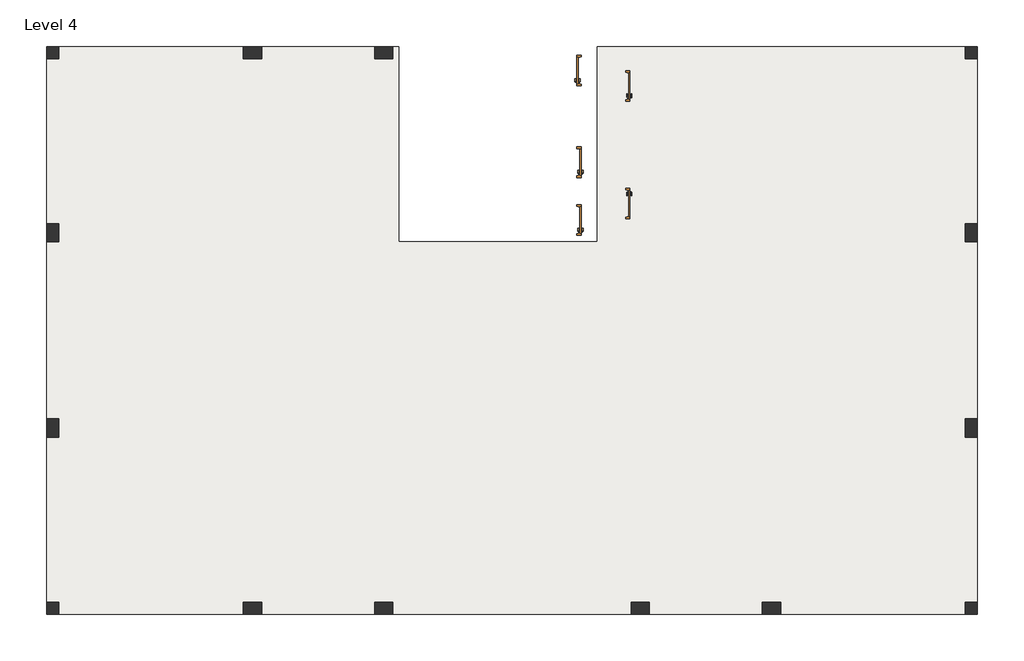
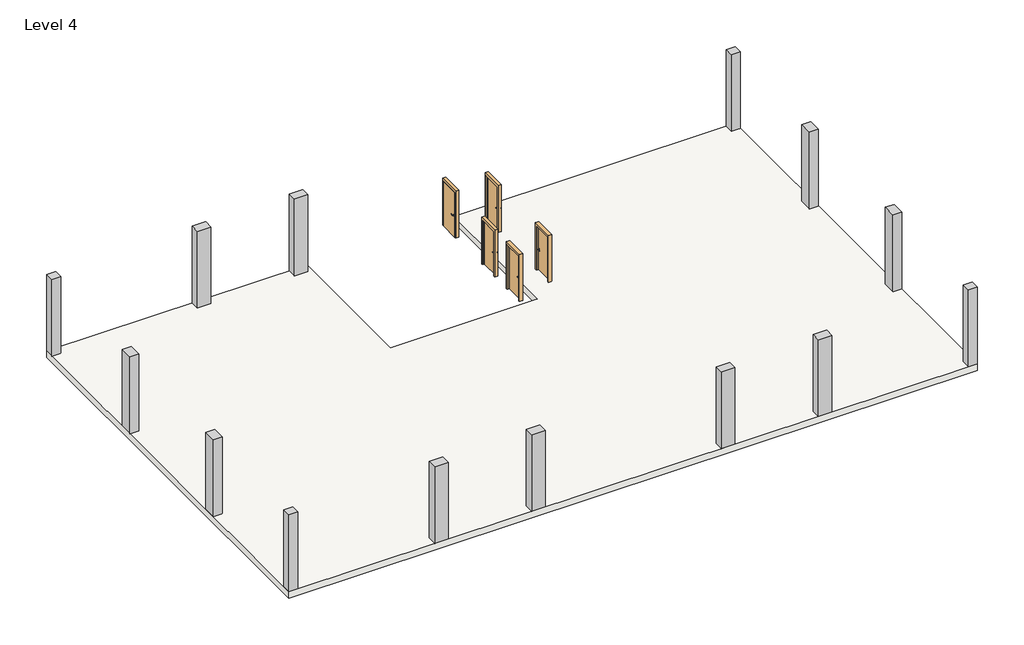
# One storey: 14 columns, 5 doors, 1 slab.
"""IFC4 building model written with IfcOpenShell, lengths in millimetres."""

import ifcopenshell
import ifcopenshell.guid

model = None  # the IFC model being written
_history = None  # IfcOwnerHistory: only IFC2X3 demands one
_inside = {}  # id of a spatial element -> (the spatial element, [elements in it])
_under = {}  # id of a project, library or spatial element -> (it, [spatial elements below it])
_declared = {}  # id of a project -> (the project, [libraries it declares])
_typed = {}  # id of a type object -> (the type object, [elements of that type])
_made_of = {}  # id of a material, layer set ... -> (it, [elements and type objects made of it])


def new_model(schema):
    """Start an empty IFC model of exactly this schema.

    Asked for "IFC4X3", IfcOpenShell would pick the latest addendum, in which some entities
    have other attributes; the version numbers below select the first issue.
    IFC2X3 requires an IfcOwnerHistory on every rooted entity: one is made here for all.
    """
    global model, _history
    if schema == "IFC4X3":
        model = ifcopenshell.file(schema_version=(4, 3, 0, 0))
    else:
        model = ifcopenshell.file(schema=schema)
    _inside.clear()
    _under.clear()
    _declared.clear()
    _typed.clear()
    _made_of.clear()
    _history = None
    if model.schema == "IFC2X3":
        org = make("IfcOrganization", Name="unknown")
        user = make(
            "IfcPersonAndOrganization",
            ThePerson=make("IfcPerson", FamilyName="unknown"),
            TheOrganization=org,
        )
        app = make(
            "IfcApplication",
            ApplicationDeveloper=org,
            Version="unknown",
            ApplicationFullName="unknown",
            ApplicationIdentifier="unknown",
        )
        _history = make(
            "IfcOwnerHistory",
            OwningUser=user,
            OwningApplication=app,
            ChangeAction="ADDED",
            CreationDate=0,
        )
    return model


def make(cls, **values):
    """One entity of the class cls with the attributes given. An attribute that is None is left unset."""
    return model.create_entity(
        cls, **{name: value for name, value in values.items() if value is not None}
    )


def rooted(cls, **values):
    """An entity with a GlobalId (a new one), such as an element, a storey or a relation."""
    return make(cls, GlobalId=ifcopenshell.guid.new(), OwnerHistory=_history, **values)


def si_unit(unit_type, name, prefix=None):
    """IfcSIUnit, for example si_unit("LENGTHUNIT", "METRE", prefix="MILLI")."""
    return make("IfcSIUnit", UnitType=unit_type, Prefix=prefix, Name=name)


def assignment(units):
    """IfcUnitAssignment: the units of a project."""
    return None if units is None else make("IfcUnitAssignment", Units=units)


def point(xyz):
    """IfcCartesianPoint."""
    return None if xyz is None else make("IfcCartesianPoint", Coordinates=xyz)


def direction(xyz):
    """IfcDirection."""
    return None if xyz is None else make("IfcDirection", DirectionRatios=xyz)


def frame(location, z_axis=None, x_axis=None):
    """IfcAxis2Placement3D, a coordinate frame: its origin and axes. An axis left out is left unset."""
    return make(
        "IfcAxis2Placement3D",
        Location=point(location),
        Axis=direction(z_axis),
        RefDirection=direction(x_axis),
    )


def frame_2d(location, x_axis=None):
    """IfcAxis2Placement2D, a coordinate frame in the plane: its origin and x axis."""
    return make(
        "IfcAxis2Placement2D", Location=point(location), RefDirection=direction(x_axis)
    )


def origin():
    """The frame at (0, 0, 0) with its axes left unset."""
    return frame((0.0, 0.0, 0.0))


def origin_with_axes():
    """The frame at (0, 0, 0) with the z axis (0, 0, 1) and the x axis (1, 0, 0) written out."""
    return frame((0.0, 0.0, 0.0), z_axis=(0.0, 0.0, 1.0), x_axis=(1.0, 0.0, 0.0))


def place(relative_to, where):
    """IfcLocalPlacement: puts the frame where relative to a parent placement (None: the world)."""
    return make(
        "IfcLocalPlacement", PlacementRelTo=relative_to, RelativePlacement=where
    )


def context(
    kind, dimensions, precision=None, world=None, true_north=None, identifier=None
):
    """IfcGeometricRepresentationContext, for example the 3D "Model" context."""
    return make(
        "IfcGeometricRepresentationContext",
        ContextIdentifier=identifier,
        ContextType=kind,
        CoordinateSpaceDimension=dimensions,
        Precision=precision,
        WorldCoordinateSystem=world,
        TrueNorth=true_north,
    )


def project(units=None, contexts=None):
    """IfcProject with its units and contexts."""
    return rooted(
        "IfcProject",
        Name="project",
        RepresentationContexts=contexts,
        UnitsInContext=assignment(units),
    )


def spatial(cls, under=None, at=None, **own):
    """A site, building, storey or space (cls), placed at a placement, below another one or the project."""
    s = rooted(cls, ObjectPlacement=at, **own)
    if under is not None:
        _under.setdefault(under.id(), (under, []))[1].append(s)
    return s


def polyline(points):
    """IfcPolyline through the points."""
    return make("IfcPolyline", Points=[point(p) for p in points])


def circle_curve(where, radius):
    """IfcCircle in the frame where."""
    return make("IfcCircle", Position=where, Radius=radius)


def ellipse_curve(where, semi_axis1, semi_axis2):
    """IfcEllipse in the frame where."""
    return make(
        "IfcEllipse", Position=where, SemiAxis1=semi_axis1, SemiAxis2=semi_axis2
    )


def trimmed(basis, trim1, trim2, sense, master):
    """IfcTrimmedCurve: the piece of a basis curve between two trims."""
    return make(
        "IfcTrimmedCurve",
        BasisCurve=basis,
        Trim1=trim1,
        Trim2=trim2,
        SenseAgreement=sense,
        MasterRepresentation=master,
    )


def segment(curve, same_sense, transition):
    """IfcCompositeCurveSegment."""
    return make(
        "IfcCompositeCurveSegment",
        Transition=transition,
        SameSense=same_sense,
        ParentCurve=curve,
    )


def composite_curve(segments, self_intersect=None):
    """IfcCompositeCurve: segments joined end to end."""
    return make("IfcCompositeCurve", Segments=segments, SelfIntersect=self_intersect)


def outline(outer, holes=None, kind="AREA"):
    """IfcArbitraryClosedProfileDef: a profile drawn as a closed curve; with holes, ...WithVoids."""
    if holes is None:
        return make("IfcArbitraryClosedProfileDef", ProfileType=kind, OuterCurve=outer)
    return make(
        "IfcArbitraryProfileDefWithVoids",
        ProfileType=kind,
        OuterCurve=outer,
        InnerCurves=holes,
    )


def extrude(swept, where, along, depth):
    """IfcExtrudedAreaSolid: the profile swept, set in the frame where, extruded along a direction by depth."""
    return make(
        "IfcExtrudedAreaSolid",
        SweptArea=swept,
        Position=where,
        ExtrudedDirection=direction(along),
        Depth=depth,
    )


def faces_of(points, faces, orient=None, outer=None):
    """IfcFace entities. A face is a list of loops; a loop is a list of indices into points, from 0.

    orient and outer hold one flag for each loop. By default every Orientation is true, the
    first loop of a face is its IfcFaceOuterBound and the others are IfcFaceBound.
    """
    made = []
    for i, loops in enumerate(faces):
        bounds = []
        for j, loop in enumerate(loops):
            is_outer = j == 0 if outer is None else outer[i][j]
            bounds.append(
                make(
                    "IfcFaceOuterBound" if is_outer else "IfcFaceBound",
                    Bound=make("IfcPolyLoop", Polygon=[points[k] for k in loop]),
                    Orientation=True if orient is None else orient[i][j],
                )
            )
        made.append(make("IfcFace", Bounds=bounds))
    return made


def faceted_brep(points, faces, orient=None, outer=None, voids=None):
    """IfcFacetedBrep: a solid bounded by flat faces; with voids (closed shells), ...WithVoids."""
    shared = [point(p) for p in points]
    hull = make("IfcClosedShell", CfsFaces=faces_of(shared, faces, orient, outer))
    if voids is None:
        return make("IfcFacetedBrep", Outer=hull)
    return make(
        "IfcFacetedBrepWithVoids",
        Outer=hull,
        Voids=[
            make(cls, CfsFaces=faces_of(shared, fs, o, b)) for cls, fs, o, b in voids
        ],
    )


def shape(context_of_items, identifier, shape_type, items):
    """IfcShapeRepresentation: the items that make up one representation, for example the "Body"."""
    return make(
        "IfcShapeRepresentation",
        ContextOfItems=context_of_items,
        RepresentationIdentifier=identifier,
        RepresentationType=shape_type,
        Items=items,
    )


def source(mapping_origin, context_of_items, identifier, shape_type, items):
    """IfcRepresentationMap: a shape defined once, which mapped items show again and again."""
    return make(
        "IfcRepresentationMap",
        MappingOrigin=mapping_origin,
        MappedRepresentation=shape(context_of_items, identifier, shape_type, items),
    )


def transform(
    local_origin,
    x_axis=None,
    y_axis=None,
    z_axis=None,
    scale=None,
    scale2=None,
    scale3=None,
    uniform=True,
):
    """IfcCartesianTransformationOperator3D, or its non-uniform kind. x_axis, y_axis, z_axis: its Axis1, 2, 3."""
    if uniform:
        return make(
            "IfcCartesianTransformationOperator3D",
            Axis1=direction(x_axis),
            Axis2=direction(y_axis),
            LocalOrigin=point(local_origin),
            Scale=scale,
            Axis3=direction(z_axis),
        )
    return make(
        "IfcCartesianTransformationOperator3DnonUniform",
        Axis1=direction(x_axis),
        Axis2=direction(y_axis),
        LocalOrigin=point(local_origin),
        Scale=scale,
        Axis3=direction(z_axis),
        Scale2=scale2,
        Scale3=scale3,
    )


def mapped(mapping_source, mapping_target):
    """IfcMappedItem: shows the shape of a source again, moved by a transform."""
    return make(
        "IfcMappedItem", MappingSource=mapping_source, MappingTarget=mapping_target
    )


def made_of(thing, what):
    """Note that an element or type object is made of a material, layer set ...; save() writes the relation."""
    if what is not None:
        _made_of.setdefault(what.id(), (what, []))[1].append(thing)
    return thing


def element(
    cls,
    number,
    at=None,
    inside=None,
    cuts=None,
    type_object=None,
    material=None,
    context=None,
    identifier="Body",
    shape_type=None,
    held_by="IfcProductDefinitionShape",
    body=None,
    shapes=None,
    **own,
):
    """One element of the class cls, such as IfcWall. Its Tag is "e" and its number.

    at: its placement. inside: the storey or other place that contains it. cuts: it is an
    opening in that element (IfcRelVoidsElement). A single representation is given by context,
    identifier, shape_type and body (its items); several are given by shapes. held_by: the class
    of the entity that holds the representations. save() writes the other relations.
    """
    e = rooted(cls, Tag="e%d" % number, ObjectPlacement=at, **own)
    if body is not None:
        shapes = [shape(context, identifier, shape_type, body)]
    if shapes is not None:
        e.Representation = make(held_by, Representations=shapes)
    if inside is not None:
        _inside.setdefault(inside.id(), (inside, []))[1].append(e)
    if cuts is not None:
        rooted(
            "IfcRelVoidsElement", RelatingBuildingElement=cuts, RelatedOpeningElement=e
        )
    if type_object is not None:
        _typed.setdefault(type_object.id(), (type_object, []))[1].append(e)
    return made_of(e, material)


def aggregate(whole, parts):
    """IfcRelAggregates: a whole, such as a stair, and the parts it consists of."""
    return rooted("IfcRelAggregates", RelatingObject=whole, RelatedObjects=parts)


def save(model, path):
    """Write the relations noted so far, then the file.

    IfcRelAggregates (storeys below a building ...), IfcRelContainedInSpatialStructure (elements
    in a storey), IfcRelDefinesByType, IfcRelAssociatesMaterial and IfcRelDeclares: one each for
    every whole, place, type object, material and project.
    """
    for whole, parts in _under.values():
        aggregate(whole, parts)
    for where, things in _inside.values():
        rooted(
            "IfcRelContainedInSpatialStructure",
            RelatedElements=things,
            RelatingStructure=where,
        )
    for kind, things in _typed.values():
        rooted("IfcRelDefinesByType", RelatedObjects=things, RelatingType=kind)
    for what, things in _made_of.values():
        rooted("IfcRelAssociatesMaterial", RelatedObjects=things, RelatingMaterial=what)
    for by, libraries in _declared.values():
        rooted("IfcRelDeclares", RelatingContext=by, RelatedDefinitions=libraries)
    model.write(path)


def plane_surface(at):
    """IfcPlane: the flat surface through the origin of the frame at, square to its z axis."""
    return make("IfcPlane", Position=at)


def cylinder_surface(at, radius):
    """IfcCylindricalSurface: all points at the distance radius from the z axis of the frame at."""
    return make("IfcCylindricalSurface", Position=at, Radius=radius)


def revolved_surface(curve, axis_point, axis_direction):
    """IfcSurfaceOfRevolution: the curve turned about the line through axis_point along axis_direction."""
    return make(
        "IfcSurfaceOfRevolution",
        SweptCurve=make("IfcArbitraryOpenProfileDef", ProfileType="CURVE", Curve=curve),
        AxisPosition=make("IfcAxis1Placement", Location=point(axis_point), Axis=direction(axis_direction)),
    )


def advanced_brep(points, edges, surfaces, faces):
    """IfcAdvancedBrep: a solid bounded by faces that lie on surfaces and meet in shared edges.

    An edge is (start, end): straight between two places in points (the first is 0);
    or (start, end, curve); or (start, end, curve, False) where it runs against its curve.
    A face is (place in surfaces, loops), or (place, loops, False) where it looks against
    its surface's normal. A loop lists edges by number (the first is 1), with a minus sign
    where the edge is run from its end to its start. The first loop is the outer one.
    """
    corners = [point(p) for p in points]
    vertices = [make("IfcVertexPoint", VertexGeometry=c) for c in corners]
    made = []
    for start, end, *more in edges:
        made.append(
            make(
                "IfcEdgeCurve",
                EdgeStart=vertices[start],
                EdgeEnd=vertices[end],
                EdgeGeometry=more[0] if more else make("IfcPolyline", Points=[corners[start], corners[end]]),
                SameSense=more[1] if len(more) > 1 else True,
            )
        )
    hull = []
    for where, loops, *sense in faces:
        bounds = []
        for j, loop in enumerate(loops):
            ring = [make("IfcOrientedEdge", EdgeElement=made[abs(k) - 1], Orientation=k > 0) for k in loop]
            bounds.append(
                make(
                    "IfcFaceOuterBound" if j == 0 else "IfcFaceBound",
                    Bound=make("IfcEdgeLoop", EdgeList=ring),
                    Orientation=True,
                )
            )
        hull.append(make("IfcAdvancedFace", Bounds=bounds, FaceSurface=surfaces[where], SameSense=sense[0] if sense else True))
    return make("IfcAdvancedBrep", Outer=make("IfcClosedShell", CfsFaces=hull))


def door_9f6fe377(model_context):
    return source(origin(), model_context, "Body", "SolidModel", [
        advanced_brep(
        [(-392.190625, -25.3375, 1016.0), (-372.190625, -25.3375, 1016.0), (-392.190625, 4.6625, 1016.0), (-372.190625, 4.6625, 1016.0), (-367.190625, 9.6625, 1016.0), (-367.190625, 29.6625, 1016.0), (-262.190625, 29.6625, 1016.0), (-262.190625, 9.6625, 1016.0)],
        [
            (0, 1, circle_curve(frame((-382.190625, -25.3375, 1016.0), z_axis=(0.0, -1.0, 0.0), x_axis=(1.0, 0.0, 0.0)), 10.0)),
            (1, 0, circle_curve(frame((-382.190625, -25.3375, 1016.0), z_axis=(0.0, -1.0, 0.0), x_axis=(1.0, 0.0, 0.0)), 10.0)),
            (0, 2),
            (2, 3, circle_curve(frame((-382.190625, 4.6625, 1016.0), z_axis=(0.0, -1.0, 0.0), x_axis=(1.0, 0.0, 0.0)), 10.0)),
            (3, 1),
            (3, 2, circle_curve(frame((-382.190625, 4.6625, 1016.0), z_axis=(0.0, -1.0, 0.0), x_axis=(1.0, 0.0, 0.0)), 10.0)),
            (4, 3, circle_curve(frame((-367.190625, 4.6625, 1016.0), z_axis=(0.0, 0.0, 1.0), x_axis=(-1.0, 0.0, 0.0)), 5.0)),
            (2, 5, circle_curve(frame((-367.190625, 4.6625, 1016.0), z_axis=(0.0, 0.0, -1.0), x_axis=(-1.0, 0.0, 0.0)), 25.0)),
            (5, 4, circle_curve(frame((-367.190625, 19.6625, 1016.0), z_axis=(-1.0, 0.0, 0.0), x_axis=(0.0, -1.0, 0.0)), 10.0)),
            (4, 5, circle_curve(frame((-367.190625, 19.6625, 1016.0), z_axis=(-1.0, 0.0, 0.0), x_axis=(0.0, -1.0, 0.0)), 10.0)),
            (6, 7, circle_curve(frame((-262.190625, 19.6625, 1016.0), z_axis=(1.0, 0.0, 0.0), x_axis=(0.0, -1.0, 0.0)), 10.0)),
            (7, 6, circle_curve(frame((-262.190625, 19.6625, 1016.0), z_axis=(1.0, 0.0, 0.0), x_axis=(0.0, -1.0, 0.0)), 10.0)),
            (5, 6),
            (7, 4),
        ],
        [
            plane_surface(frame((-382.190625, -25.3375, 1016.0), z_axis=(0.0, -1.0, 0.0), x_axis=(0.0, 0.0, 1.0))),
            cylinder_surface(frame((-382.190625, -25.3375, 1016.0), z_axis=(0.0, -1.0, 0.0), x_axis=(1.0, 0.0, 0.0)), 10.0),
            revolved_surface(trimmed(ellipse_curve(frame((-382.190625, 4.6625, 1016.0), z_axis=(0.0, -1.0, 0.0), x_axis=(1.0, 0.0, 0.0)), 10.0, 10.0), [point((-392.190625, 4.6625, 1016.0))], [point((-372.190625, 4.6625, 1016.0))], True, "CARTESIAN"), (-367.190625, 4.6625, 1016.0), (0.0, 0.0, -1.0)),
            revolved_surface(trimmed(ellipse_curve(frame((-382.190625, 4.6625, 1016.0), z_axis=(0.0, -1.0, 0.0), x_axis=(1.0, 0.0, 0.0)), 10.0, 10.0), [point((-372.190625, 4.6625, 1016.0))], [point((-392.190625, 4.6625, 1016.0))], True, "CARTESIAN"), (-367.190625, 4.6625, 1016.0), (0.0, 0.0, -1.0)),
            plane_surface(frame((-262.190625, 19.6625, 1016.0), z_axis=(1.0, 0.0, 0.0), x_axis=(0.0, 0.0, 1.0))),
            cylinder_surface(frame((-367.190625, 19.6625, 1016.0), z_axis=(-1.0, 0.0, 0.0), x_axis=(0.0, -1.0, 0.0)), 10.0),
        ],
        [
            (0, [[1, 2]]),
            (1, [[-1, 3, 4, 5]]),
            (1, [[-2, -5, 6, -3]]),
            (2, [[7, -4, 8, 9]]),
            (3, [[-8, -6, -7, 10]]),
            (4, [[11, 12]]),
            (5, [[-9, 13, -12, 14]]),
            (5, [[-10, -14, -11, -13]]),
        ],
    ),
        extrude(outline(composite_curve([segment(trimmed(circle_curve(frame_2d((1016.0, -384.690625)), 30.0), [point((1016.0, -414.690625))], [point((1016.0, -354.690625))], False, "CARTESIAN"), True, "CONTINUOUS"), segment(trimmed(circle_curve(frame_2d((1016.0, -384.690625)), 30.0), [point((1016.0, -354.690625))], [point((1016.0, -414.690625))], False, "CARTESIAN"), True, "CONTINUOUS")], self_intersect=False)), frame((0.0, -33.3375, 0.0), z_axis=(0.0, 1.0, 0.0), x_axis=(0.0, 0.0, 1.0)), (0.0, 0.0, 1.0), 8.0),
        advanced_brep(
        [(-392.190625, -85.7875, 1016.0), (-372.190625, -85.7875, 1016.0), (-372.190625, -115.7875, 1016.0), (-392.190625, -115.7875, 1016.0), (-367.190625, -120.7875, 1016.0), (-367.190625, -140.7875, 1016.0), (-262.190625, -140.7875, 1016.0), (-262.190625, -120.7875, 1016.0)],
        [
            (0, 1, circle_curve(frame((-382.190625, -85.7875, 1016.0), z_axis=(0.0, 1.0, 0.0), x_axis=(1.0, 0.0, 0.0)), 10.0)),
            (1, 0, circle_curve(frame((-382.190625, -85.7875, 1016.0), z_axis=(0.0, 1.0, 0.0), x_axis=(1.0, 0.0, 0.0)), 10.0)),
            (1, 2),
            (2, 3, circle_curve(frame((-382.190625, -115.7875, 1016.0), z_axis=(0.0, 1.0, 0.0), x_axis=(1.0, 0.0, 0.0)), 10.0)),
            (3, 0),
            (3, 2, circle_curve(frame((-382.190625, -115.7875, 1016.0), z_axis=(0.0, 1.0, 0.0), x_axis=(1.0, 0.0, 0.0)), 10.0)),
            (4, 5, circle_curve(frame((-367.190625, -130.7875, 1016.0), z_axis=(-1.0, 0.0, 0.0), x_axis=(0.0, 1.0, 0.0)), 10.0)),
            (5, 3, circle_curve(frame((-367.190625, -115.7875, 1016.0), z_axis=(0.0, 0.0, -1.0), x_axis=(-1.0, 0.0, 0.0)), 25.0)),
            (2, 4, circle_curve(frame((-367.190625, -115.7875, 1016.0), z_axis=(0.0, 0.0, 1.0), x_axis=(-1.0, 0.0, 0.0)), 5.0)),
            (5, 4, circle_curve(frame((-367.190625, -130.7875, 1016.0), z_axis=(-1.0, 0.0, 0.0), x_axis=(0.0, 1.0, 0.0)), 10.0)),
            (6, 7, circle_curve(frame((-262.190625, -130.7875, 1016.0), z_axis=(1.0, 0.0, 0.0), x_axis=(0.0, 1.0, 0.0)), 10.0)),
            (7, 6, circle_curve(frame((-262.190625, -130.7875, 1016.0), z_axis=(1.0, 0.0, 0.0), x_axis=(0.0, 1.0, 0.0)), 10.0)),
            (4, 7),
            (6, 5),
        ],
        [
            plane_surface(frame((-382.190625, -85.7875, 1016.0), z_axis=(0.0, 1.0, 0.0), x_axis=(0.0, 0.0, 1.0))),
            cylinder_surface(frame((-382.190625, -85.7875, 1016.0), z_axis=(0.0, 1.0, 0.0), x_axis=(1.0, 0.0, 0.0)), 10.0),
            revolved_surface(trimmed(ellipse_curve(frame((-382.190625, -115.7875, 1016.0), z_axis=(0.0, -1.0, 0.0), x_axis=(1.0, 0.0, 0.0)), 10.0, 10.0), [point((-392.190625, -115.7875, 1016.0))], [point((-372.190625, -115.7875, 1016.0))], True, "CARTESIAN"), (-367.190625, -115.7875, 1016.0), (0.0, 0.0, -1.0)),
            revolved_surface(trimmed(ellipse_curve(frame((-382.190625, -115.7875, 1016.0), z_axis=(0.0, -1.0, 0.0), x_axis=(1.0, 0.0, 0.0)), 10.0, 10.0), [point((-372.190625, -115.7875, 1016.0))], [point((-392.190625, -115.7875, 1016.0))], True, "CARTESIAN"), (-367.190625, -115.7875, 1016.0), (0.0, 0.0, -1.0)),
            plane_surface(frame((-262.190625, -130.7875, 1016.0), z_axis=(1.0, 0.0, 0.0), x_axis=(0.0, 0.0, 1.0))),
            cylinder_surface(frame((-367.190625, -130.7875, 1016.0), z_axis=(-1.0, 0.0, 0.0), x_axis=(0.0, 1.0, 0.0)), 10.0),
        ],
        [
            (0, [[1, 2]]),
            (1, [[3, 4, 5, -2]]),
            (1, [[-5, 6, -3, -1]]),
            (2, [[7, 8, -4, 9]]),
            (3, [[10, -9, -6, -8]]),
            (4, [[11, 12]]),
            (5, [[13, -11, 14, -7]]),
            (5, [[-14, -12, -13, -10]]),
        ],
    ),
        extrude(outline(composite_curve([segment(trimmed(circle_curve(frame_2d((1016.0, -384.690625)), 30.0), [point((1016.0, -414.690625))], [point((1016.0, -354.690625))], False, "CARTESIAN"), True, "CONTINUOUS"), segment(trimmed(circle_curve(frame_2d((1016.0, -384.690625)), 30.0), [point((1016.0, -354.690625))], [point((1016.0, -414.690625))], False, "CARTESIAN"), True, "CONTINUOUS")], self_intersect=False)), frame((0.0, -85.7875, 0.0), z_axis=(0.0, 1.0, 0.0), x_axis=(0.0, 0.0, 1.0)), (0.0, 0.0, 1.0), 8.0),
        faceted_brep([(457.2, -28.575, 0.0), (441.325, -28.575, 0.0), (441.325, 19.05, 0.0), (457.2, 19.05, 0.0), (457.2, 68.2625, 0.0), (508.0, 68.2625, 0.0), (508.0, -77.7875, 0.0), (457.2, -77.7875, 0.0), (457.2, -77.7875, 2133.6), (457.2, -28.575, 2133.6), (508.0, -77.7875, 2235.2), (-508.0, -77.7875, 2235.2), (-508.0, -77.7875, 0.0), (-457.2, -77.7875, 0.0), (-457.2, -77.7875, 2133.6), (508.0, 68.2625, 2235.2), (457.2, 68.2625, 2133.6), (-457.2, 68.2625, 2133.6), (-457.2, 68.2625, 0.0), (-508.0, 68.2625, 0.0), (-508.0, 68.2625, 2235.2), (457.2, 19.05, 2133.6), (441.325, 19.05, 2117.725), (-441.325, 19.05, 2117.725), (-441.325, 19.05, 0.0), (-457.2, 19.05, 0.0), (-457.2, 19.05, 2133.6), (441.325, -28.575, 2117.725), (-457.2, -28.575, 2133.6), (-457.2, -28.575, 0.0), (-441.325, -28.575, 0.0), (-441.325, -28.575, 2117.725)], [[[0, 1, 2, 3, 4, 5, 6, 7]], [[7, 8, 9, 0]], [[6, 10, 11, 12, 13, 14, 8, 7]], [[5, 15, 10, 6]], [[4, 16, 17, 18, 19, 20, 15, 5]], [[3, 21, 16, 4]], [[2, 22, 23, 24, 25, 26, 21, 3]], [[1, 27, 22, 2]], [[0, 9, 28, 29, 30, 31, 27, 1]], [[8, 14, 28, 9]], [[16, 21, 26, 17]], [[22, 27, 31, 23]], [[12, 19, 18, 25, 24, 30, 29, 13]], [[13, 29, 28, 14]], [[11, 20, 19, 12]], [[17, 26, 25, 18]], [[23, 31, 30, 24]], [[15, 20, 11, 10]]]),
        extrude(outline(polyline([(457.2, -33.3375), (457.2, -77.7875), (-457.2, -77.7875), (-457.2, -33.3375), (457.2, -33.3375)])), origin_with_axes(), (0.0, 0.0, 1.0), 2133.6),
    ])


def door_87fe937e(model_context):
    return source(origin(), model_context, "Body", "SolidModel", [
        advanced_brep(
        [(-392.190625, 25.3375, 1016.0), (-372.190625, 25.3375, 1016.0), (-372.190625, -4.6625, 1016.0), (-392.190625, -4.6625, 1016.0), (-367.190625, -9.6625, 1016.0), (-367.190625, -29.6625, 1016.0), (-262.190625, -29.6625, 1016.0), (-262.190625, -9.6625, 1016.0)],
        [
            (0, 1, circle_curve(frame((-382.190625, 25.3375, 1016.0), z_axis=(0.0, 1.0, 0.0), x_axis=(1.0, 0.0, 0.0)), 10.0)),
            (1, 0, circle_curve(frame((-382.190625, 25.3375, 1016.0), z_axis=(0.0, 1.0, 0.0), x_axis=(1.0, 0.0, 0.0)), 10.0)),
            (1, 2),
            (2, 3, circle_curve(frame((-382.190625, -4.6625, 1016.0), z_axis=(0.0, 1.0, 0.0), x_axis=(1.0, 0.0, 0.0)), 10.0)),
            (3, 0),
            (3, 2, circle_curve(frame((-382.190625, -4.6625, 1016.0), z_axis=(0.0, 1.0, 0.0), x_axis=(1.0, 0.0, 0.0)), 10.0)),
            (4, 5, circle_curve(frame((-367.190625, -19.6625, 1016.0), z_axis=(-1.0, 0.0, 0.0), x_axis=(0.0, 1.0, 0.0)), 10.0)),
            (5, 3, circle_curve(frame((-367.190625, -4.6625, 1016.0), z_axis=(0.0, 0.0, -1.0), x_axis=(-1.0, 0.0, 0.0)), 25.0)),
            (2, 4, circle_curve(frame((-367.190625, -4.6625, 1016.0), z_axis=(0.0, 0.0, 1.0), x_axis=(-1.0, 0.0, 0.0)), 5.0)),
            (5, 4, circle_curve(frame((-367.190625, -19.6625, 1016.0), z_axis=(-1.0, 0.0, 0.0), x_axis=(0.0, 1.0, 0.0)), 10.0)),
            (6, 7, circle_curve(frame((-262.190625, -19.6625, 1016.0), z_axis=(1.0, 0.0, 0.0), x_axis=(0.0, 1.0, 0.0)), 10.0)),
            (7, 6, circle_curve(frame((-262.190625, -19.6625, 1016.0), z_axis=(1.0, 0.0, 0.0), x_axis=(0.0, 1.0, 0.0)), 10.0)),
            (4, 7),
            (6, 5),
        ],
        [
            plane_surface(frame((-382.190625, 25.3375, 1016.0), z_axis=(0.0, 1.0, 0.0), x_axis=(0.0, 0.0, 1.0))),
            cylinder_surface(frame((-382.190625, 25.3375, 1016.0), z_axis=(0.0, 1.0, 0.0), x_axis=(1.0, 0.0, 0.0)), 10.0),
            revolved_surface(trimmed(ellipse_curve(frame((-382.190625, -4.6625, 1016.0), z_axis=(0.0, -1.0, 0.0), x_axis=(1.0, 0.0, 0.0)), 10.0, 10.0), [point((-392.190625, -4.6625, 1016.0))], [point((-372.190625, -4.6625, 1016.0))], True, "CARTESIAN"), (-367.190625, -4.6625, 1016.0), (0.0, 0.0, -1.0)),
            revolved_surface(trimmed(ellipse_curve(frame((-382.190625, -4.6625, 1016.0), z_axis=(0.0, -1.0, 0.0), x_axis=(1.0, 0.0, 0.0)), 10.0, 10.0), [point((-372.190625, -4.6625, 1016.0))], [point((-392.190625, -4.6625, 1016.0))], True, "CARTESIAN"), (-367.190625, -4.6625, 1016.0), (0.0, 0.0, -1.0)),
            plane_surface(frame((-262.190625, -19.6625, 1016.0), z_axis=(1.0, 0.0, 0.0), x_axis=(0.0, 0.0, 1.0))),
            cylinder_surface(frame((-367.190625, -19.6625, 1016.0), z_axis=(-1.0, 0.0, 0.0), x_axis=(0.0, 1.0, 0.0)), 10.0),
        ],
        [
            (0, [[1, 2]]),
            (1, [[3, 4, 5, -2]]),
            (1, [[-5, 6, -3, -1]]),
            (2, [[7, 8, -4, 9]]),
            (3, [[10, -9, -6, -8]]),
            (4, [[11, 12]]),
            (5, [[13, -11, 14, -7]]),
            (5, [[-14, -12, -13, -10]]),
        ],
    ),
        extrude(outline(composite_curve([segment(trimmed(circle_curve(frame_2d((1016.0, -384.690625)), 30.0), [point((1016.0, -414.690625))], [point((1016.0, -354.690625))], False, "CARTESIAN"), True, "CONTINUOUS"), segment(trimmed(circle_curve(frame_2d((1016.0, -384.690625)), 30.0), [point((1016.0, -354.690625))], [point((1016.0, -414.690625))], False, "CARTESIAN"), True, "CONTINUOUS")], self_intersect=False)), frame((0.0, 25.3375, 0.0), z_axis=(0.0, 1.0, 0.0), x_axis=(0.0, 0.0, 1.0)), (0.0, 0.0, 1.0), 8.0),
        advanced_brep(
        [(-392.190625, 85.7875, 1016.0), (-372.190625, 85.7875, 1016.0), (-392.190625, 115.7875, 1016.0), (-372.190625, 115.7875, 1016.0), (-367.190625, 120.7875, 1016.0), (-367.190625, 140.7875, 1016.0), (-262.190625, 140.7875, 1016.0), (-262.190625, 120.7875, 1016.0)],
        [
            (0, 1, circle_curve(frame((-382.190625, 85.7875, 1016.0), z_axis=(0.0, -1.0, 0.0), x_axis=(1.0, 0.0, 0.0)), 10.0)),
            (1, 0, circle_curve(frame((-382.190625, 85.7875, 1016.0), z_axis=(0.0, -1.0, 0.0), x_axis=(1.0, 0.0, 0.0)), 10.0)),
            (0, 2),
            (2, 3, circle_curve(frame((-382.190625, 115.7875, 1016.0), z_axis=(0.0, -1.0, 0.0), x_axis=(1.0, 0.0, 0.0)), 10.0)),
            (3, 1),
            (3, 2, circle_curve(frame((-382.190625, 115.7875, 1016.0), z_axis=(0.0, -1.0, 0.0), x_axis=(1.0, 0.0, 0.0)), 10.0)),
            (4, 3, circle_curve(frame((-367.190625, 115.7875, 1016.0), z_axis=(0.0, 0.0, 1.0), x_axis=(-1.0, 0.0, 0.0)), 5.0)),
            (2, 5, circle_curve(frame((-367.190625, 115.7875, 1016.0), z_axis=(0.0, 0.0, -1.0), x_axis=(-1.0, 0.0, 0.0)), 25.0)),
            (5, 4, circle_curve(frame((-367.190625, 130.7875, 1016.0), z_axis=(-1.0, 0.0, 0.0), x_axis=(0.0, -1.0, 0.0)), 10.0)),
            (4, 5, circle_curve(frame((-367.190625, 130.7875, 1016.0), z_axis=(-1.0, 0.0, 0.0), x_axis=(0.0, -1.0, 0.0)), 10.0)),
            (6, 7, circle_curve(frame((-262.190625, 130.7875, 1016.0), z_axis=(1.0, 0.0, 0.0), x_axis=(0.0, -1.0, 0.0)), 10.0)),
            (7, 6, circle_curve(frame((-262.190625, 130.7875, 1016.0), z_axis=(1.0, 0.0, 0.0), x_axis=(0.0, -1.0, 0.0)), 10.0)),
            (5, 6),
            (7, 4),
        ],
        [
            plane_surface(frame((-382.190625, 85.7875, 1016.0), z_axis=(0.0, -1.0, 0.0), x_axis=(0.0, 0.0, 1.0))),
            cylinder_surface(frame((-382.190625, 85.7875, 1016.0), z_axis=(0.0, -1.0, 0.0), x_axis=(1.0, 0.0, 0.0)), 10.0),
            revolved_surface(trimmed(ellipse_curve(frame((-382.190625, 115.7875, 1016.0), z_axis=(0.0, -1.0, 0.0), x_axis=(1.0, 0.0, 0.0)), 10.0, 10.0), [point((-392.190625, 115.7875, 1016.0))], [point((-372.190625, 115.7875, 1016.0))], True, "CARTESIAN"), (-367.190625, 115.7875, 1016.0), (0.0, 0.0, -1.0)),
            revolved_surface(trimmed(ellipse_curve(frame((-382.190625, 115.7875, 1016.0), z_axis=(0.0, -1.0, 0.0), x_axis=(1.0, 0.0, 0.0)), 10.0, 10.0), [point((-372.190625, 115.7875, 1016.0))], [point((-392.190625, 115.7875, 1016.0))], True, "CARTESIAN"), (-367.190625, 115.7875, 1016.0), (0.0, 0.0, -1.0)),
            plane_surface(frame((-262.190625, 130.7875, 1016.0), z_axis=(1.0, 0.0, 0.0), x_axis=(0.0, 0.0, 1.0))),
            cylinder_surface(frame((-367.190625, 130.7875, 1016.0), z_axis=(-1.0, 0.0, 0.0), x_axis=(0.0, -1.0, 0.0)), 10.0),
        ],
        [
            (0, [[1, 2]]),
            (1, [[-1, 3, 4, 5]]),
            (1, [[-2, -5, 6, -3]]),
            (2, [[7, -4, 8, 9]]),
            (3, [[-8, -6, -7, 10]]),
            (4, [[11, 12]]),
            (5, [[-9, 13, -12, 14]]),
            (5, [[-10, -14, -11, -13]]),
        ],
    ),
        extrude(outline(composite_curve([segment(trimmed(circle_curve(frame_2d((1016.0, -384.690625)), 30.0), [point((1016.0, -414.690625))], [point((1016.0, -354.690625))], False, "CARTESIAN"), True, "CONTINUOUS"), segment(trimmed(circle_curve(frame_2d((1016.0, -384.690625)), 30.0), [point((1016.0, -354.690625))], [point((1016.0, -414.690625))], False, "CARTESIAN"), True, "CONTINUOUS")], self_intersect=False)), frame((0.0, 77.7875, 0.0), z_axis=(0.0, 1.0, 0.0), x_axis=(0.0, 0.0, 1.0)), (0.0, 0.0, 1.0), 8.0),
        faceted_brep([(457.2, 28.575, 0.0), (457.2, 77.7875, 0.0), (508.0, 77.7875, 0.0), (508.0, -68.2625, 0.0), (457.2, -68.2625, 0.0), (457.2, -19.05, 0.0), (441.325, -19.05, 0.0), (441.325, 28.575, 0.0), (457.2, 28.575, 2133.6), (457.2, 77.7875, 2133.6), (-457.2, 77.7875, 2133.6), (-457.2, 77.7875, 0.0), (-508.0, 77.7875, 0.0), (-508.0, 77.7875, 2235.2), (508.0, 77.7875, 2235.2), (508.0, -68.2625, 2235.2), (-508.0, -68.2625, 2235.2), (-508.0, -68.2625, 0.0), (-457.2, -68.2625, 0.0), (-457.2, -68.2625, 2133.6), (457.2, -68.2625, 2133.6), (457.2, -19.05, 2133.6), (-457.2, -19.05, 2133.6), (-457.2, -19.05, 0.0), (-441.325, -19.05, 0.0), (-441.325, -19.05, 2117.725), (441.325, -19.05, 2117.725), (441.325, 28.575, 2117.725), (-441.325, 28.575, 2117.725), (-441.325, 28.575, 0.0), (-457.2, 28.575, 0.0), (-457.2, 28.575, 2133.6)], [[[0, 1, 2, 3, 4, 5, 6, 7]], [[1, 0, 8, 9]], [[2, 1, 9, 10, 11, 12, 13, 14]], [[3, 2, 14, 15]], [[4, 3, 15, 16, 17, 18, 19, 20]], [[5, 4, 20, 21]], [[6, 5, 21, 22, 23, 24, 25, 26]], [[7, 6, 26, 27]], [[0, 7, 27, 28, 29, 30, 31, 8]], [[9, 8, 31, 10]], [[20, 19, 22, 21]], [[26, 25, 28, 27]], [[12, 11, 30, 29, 24, 23, 18, 17]], [[11, 10, 31, 30]], [[13, 12, 17, 16]], [[19, 18, 23, 22]], [[25, 24, 29, 28]], [[15, 14, 13, 16]]]),
        extrude(outline(polyline([(457.2, 33.3375), (-457.2, 33.3375), (-457.2, 77.7875), (457.2, 77.7875), (457.2, 33.3375)])), origin_with_axes(), (0.0, 0.0, 1.0), 2133.6),
    ])


model = new_model("IFC4")

# Units and contexts
model_context = context("Model", 3, world=origin())
ifc_project = project(units=[si_unit("LENGTHUNIT", "METRE", prefix="MILLI")], contexts=[model_context])

# Site, building, storey
site = spatial("IfcSite", under=ifc_project)
building = spatial("IfcBuilding", under=site)
storey = spatial("IfcBuildingStorey", under=building, Name="Level 4", Elevation=10972.8)

# Columns
placement = place(None, origin())
element("IfcColumn", 1, ObjectType="Rectangular Column : 24\" x 24\"", at=placement, inside=storey, context=model_context, shape_type="SweptSolid", body=[
    extrude(outline(polyline([(-16253.4122732, 9291.5015304), (-16253.4122732, 8885.1015304), (-16659.8122732, 8885.1015304), (-16659.8122732, 9291.5015304), (-16253.4122732, 9291.5015304)])), frame((0.0, 0.0, 10972.8), z_axis=(0.0, 0.0, 1.0), x_axis=(1.0, 0.0, 0.0)), (0.0, 0.0, 1.0), 3657.6),
])
element("IfcColumn", 2, ObjectType="Rectangular Column : 24\" x 24\"", at=placement, inside=storey, context=model_context, shape_type="SweptSolid", body=[
    extrude(outline(polyline([(-16253.4122732, 3398.7015304), (-16253.4122732, 2789.1015304), (-16659.8122732, 2789.1015304), (-16659.8122732, 3398.7015304), (-16253.4122732, 3398.7015304)])), frame((0.0, 0.0, 10972.8), z_axis=(0.0, 0.0, 1.0), x_axis=(1.0, 0.0, 0.0)), (0.0, 0.0, 1.0), 3657.6),
])
element("IfcColumn", 3, ObjectType="Rectangular Column : 24\" x 24\"", at=placement, inside=storey, context=model_context, shape_type="SweptSolid", body=[
    extrude(outline(polyline([(-9497.0122732, 8885.1015304), (-10106.6122732, 8885.1015304), (-10106.6122732, 9291.5015304), (-9497.0122732, 9291.5015304), (-9497.0122732, 8885.1015304)])), frame((0.0, 0.0, 10972.8), z_axis=(0.0, 0.0, 1.0), x_axis=(1.0, 0.0, 0.0)), (0.0, 0.0, 1.0), 3657.6),
])
element("IfcColumn", 4, ObjectType="Rectangular Column : 24\" x 24\"", at=placement, inside=storey, context=model_context, shape_type="SweptSolid", body=[
    extrude(outline(polyline([(-5128.2122732, 8885.1015304), (-5737.8122732, 8885.1015304), (-5737.8122732, 9291.5015304), (-5128.2122732, 9291.5015304), (-5128.2122732, 8885.1015304)])), frame((0.0, 0.0, 10972.8), z_axis=(0.0, 0.0, 1.0), x_axis=(1.0, 0.0, 0.0)), (0.0, 0.0, 1.0), 3657.6),
])
element("IfcColumn", 5, ObjectType="Rectangular Column : 24\" x 24\"", at=placement, inside=storey, context=model_context, shape_type="SweptSolid", body=[
    extrude(outline(polyline([(14328.1877268, 8885.1015304), (13921.7877268, 8885.1015304), (13921.7877268, 9291.5015304), (14328.1877268, 9291.5015304), (14328.1877268, 8885.1015304)])), frame((0.0, 0.0, 10972.8), z_axis=(0.0, 0.0, 1.0), x_axis=(1.0, 0.0, 0.0)), (0.0, 0.0, 1.0), 3657.6),
])
element("IfcColumn", 6, ObjectType="Rectangular Column : 24\" x 24\"", at=placement, inside=storey, context=model_context, shape_type="SweptSolid", body=[
    extrude(outline(polyline([(13921.7877268, 2789.1015304), (13921.7877268, 3398.7015304), (14328.1877268, 3398.7015304), (14328.1877268, 2789.1015304), (13921.7877268, 2789.1015304)])), frame((0.0, 0.0, 10972.8), z_axis=(0.0, 0.0, 1.0), x_axis=(1.0, 0.0, 0.0)), (0.0, 0.0, 1.0), 3657.6),
])
element("IfcColumn", 7, ObjectType="Rectangular Column : 24\" x 24\"", at=placement, inside=storey, context=model_context, shape_type="SweptSolid", body=[
    extrude(outline(polyline([(13921.7877268, -3713.2984696), (13921.7877268, -3103.6984696), (14328.1877268, -3103.6984696), (14328.1877268, -3713.2984696), (13921.7877268, -3713.2984696)])), frame((0.0, 0.0, 10972.8), z_axis=(0.0, 0.0, 1.0), x_axis=(1.0, 0.0, 0.0)), (0.0, 0.0, 1.0), 3657.6),
])
element("IfcColumn", 8, ObjectType="Rectangular Column : 24\" x 24\"", at=placement, inside=storey, context=model_context, shape_type="SweptSolid", body=[
    extrude(outline(polyline([(13921.7877268, -9606.0984696), (13921.7877268, -9199.6984696), (14328.1877268, -9199.6984696), (14328.1877268, -9606.0984696), (13921.7877268, -9606.0984696)])), frame((0.0, 0.0, 10972.8), z_axis=(0.0, 0.0, 1.0), x_axis=(1.0, 0.0, 0.0)), (0.0, 0.0, 1.0), 3657.6),
])
element("IfcColumn", 9, ObjectType="Rectangular Column : 24\" x 24\"", at=placement, inside=storey, context=model_context, shape_type="SweptSolid", body=[
    extrude(outline(polyline([(7165.3877268, -9199.6984696), (7774.9877268, -9199.6984696), (7774.9877268, -9606.0984696), (7165.3877268, -9606.0984696), (7165.3877268, -9199.6984696)])), frame((0.0, 0.0, 10972.8), z_axis=(0.0, 0.0, 1.0), x_axis=(1.0, 0.0, 0.0)), (0.0, 0.0, 1.0), 3657.6),
])
element("IfcColumn", 10, ObjectType="Rectangular Column : 24\" x 24\"", at=placement, inside=storey, context=model_context, shape_type="SweptSolid", body=[
    extrude(outline(polyline([(2796.5877268, -9199.6984696), (3406.1877268, -9199.6984696), (3406.1877268, -9606.0984696), (2796.5877268, -9606.0984696), (2796.5877268, -9199.6984696)])), frame((0.0, 0.0, 10972.8), z_axis=(0.0, 0.0, 1.0), x_axis=(1.0, 0.0, 0.0)), (0.0, 0.0, 1.0), 3657.6),
])
element("IfcColumn", 11, ObjectType="Rectangular Column : 24\" x 24\"", at=placement, inside=storey, context=model_context, shape_type="SweptSolid", body=[
    extrude(outline(polyline([(-5737.8122732, -9199.6984696), (-5128.2122732, -9199.6984696), (-5128.2122732, -9606.0984696), (-5737.8122732, -9606.0984696), (-5737.8122732, -9199.6984696)])), frame((0.0, 0.0, 10972.8), z_axis=(0.0, 0.0, 1.0), x_axis=(1.0, 0.0, 0.0)), (0.0, 0.0, 1.0), 3657.6),
])
element("IfcColumn", 12, ObjectType="Rectangular Column : 24\" x 24\"", at=placement, inside=storey, context=model_context, shape_type="SweptSolid", body=[
    extrude(outline(polyline([(-10106.6122732, -9199.6984696), (-9497.0122732, -9199.6984696), (-9497.0122732, -9606.0984696), (-10106.6122732, -9606.0984696), (-10106.6122732, -9199.6984696)])), frame((0.0, 0.0, 10972.8), z_axis=(0.0, 0.0, 1.0), x_axis=(1.0, 0.0, 0.0)), (0.0, 0.0, 1.0), 3657.6),
])
element("IfcColumn", 13, ObjectType="Rectangular Column : 24\" x 24\"", at=placement, inside=storey, context=model_context, shape_type="SweptSolid", body=[
    extrude(outline(polyline([(-16659.8122732, -9199.6984696), (-16253.4122732, -9199.6984696), (-16253.4122732, -9606.0984696), (-16659.8122732, -9606.0984696), (-16659.8122732, -9199.6984696)])), frame((0.0, 0.0, 10972.8), z_axis=(0.0, 0.0, 1.0), x_axis=(1.0, 0.0, 0.0)), (0.0, 0.0, 1.0), 3657.6),
])
element("IfcColumn", 14, ObjectType="Rectangular Column : 24\" x 24\"", at=placement, inside=storey, context=model_context, shape_type="SweptSolid", body=[
    extrude(outline(polyline([(-16253.4122732, -3103.6984696), (-16253.4122732, -3713.2984696), (-16659.8122732, -3713.2984696), (-16659.8122732, -3103.6984696), (-16253.4122732, -3103.6984696)])), frame((0.0, 0.0, 10972.8), z_axis=(0.0, 0.0, 1.0), x_axis=(1.0, 0.0, 0.0)), (0.0, 0.0, 1.0), 3657.6),
])

# Doors
door_shape = door_9f6fe377(model_context)
element("IfcDoor", 15, ObjectType="Door-Passage-Single-Flush : 36\" x 84\"", at=placement, inside=storey, context=model_context, shape_type="MappedRepresentation", body=[
    mapped(door_shape, transform((1058.2752268, 5440.2265304, 10972.8), x_axis=(0.0, 1.0, 0.0), y_axis=(-1.0, 0.0, 0.0), z_axis=(0.0, 0.0, 1.0))),
])
element("IfcDoor", 16, ObjectType="Door-Passage-Single-Flush : 36\" x 84\"", at=placement, inside=storey, context=model_context, shape_type="MappedRepresentation", body=[
    mapped(door_shape, transform((1058.2752268, 3509.8265304, 10972.8), x_axis=(0.0, 1.0, 0.0), y_axis=(-1.0, 0.0, 0.0), z_axis=(0.0, 0.0, 1.0))),
])
element("IfcDoor", 17, ObjectType="Door-Passage-Single-Flush : 36\" x 84\"", at=placement, inside=storey, context=model_context, shape_type="MappedRepresentation", body=[
    mapped(door_shape, transform((2683.8752268, 7980.2265304, 10972.8), x_axis=(0.0, 1.0, 0.0), y_axis=(-1.0, 0.0, 0.0), z_axis=(0.0, 0.0, 1.0))),
])
door_2_shape = door_87fe937e(model_context)
element("IfcDoor", 18, ObjectType="Door-Passage-Single-Flush : 36\" x 84\"", at=placement, inside=storey, context=model_context, shape_type="MappedRepresentation", body=[
    mapped(door_2_shape, transform((1070.9752268, 8488.2265304, 10972.8), x_axis=(0.0, 1.0, 0.0), y_axis=(-1.0, 0.0, 0.0), z_axis=(0.0, 0.0, 1.0))),
])
element("IfcDoor", 19, ObjectType="Door-Passage-Single-Flush : 36\" x 84\"", at=placement, inside=storey, context=model_context, shape_type="MappedRepresentation", body=[
    mapped(door_2_shape, transform((2683.8752268, 4059.1015304, 10972.8), x_axis=(0.0, -1.0, 0.0), y_axis=(1.0, 0.0, 0.0), z_axis=(0.0, 0.0, 1.0))),
])

# Slab
element("IfcSlab", 20, ObjectType="Generic - 12\"", at=placement, inside=storey, context=model_context, shape_type="SweptSolid", body=[
    extrude(outline(polyline([(14328.1877268, 9291.5015304), (14328.1877268, -9606.0984696), (-16659.8122732, -9606.0984696), (-16659.8122732, 9291.5015304), (-4934.5372732, 9291.5015304), (-4934.5372732, 2789.1015304), (1674.2252268, 2789.1015304), (1674.2252268, 9291.5015304), (14328.1877268, 9291.5015304)])), frame((0.0, 0.0, 10668.0), z_axis=(0.0, 0.0, 1.0), x_axis=(1.0, 0.0, 0.0)), (0.0, 0.0, 1.0), 304.8),
])

save(model, "model.ifc")

# Revit data of these elements
# Type "Rectangular Column : 24\" x 24\""
#   Assembly Code = "B1010200"
#   Depth = 2' - 0"
#   Offset Base = 0' - 0"
#   Offset Top = 0' - 0"
#   Width = 2' - 0"
#   Material = none
# Type "Door-Passage-Single-Flush : 36\" x 84\""
#   Type Mark = "1"
#   Assembly Code = "B2030200"
#   Analytic Construction = "Wooden"
#   Thickness = 0' - 1 3/4"
#   Thermal Resistance (R) = 2.5876 (h·ft²·°F)/BTU
#   Swing Angle [instance default] = 90.00°
#   Strike Height = 3' - 4"
#   Rough Width [instance default] = 3' - 4"
#   Rough Height [instance default] = 7' - 4"
#   MF Opening Height [instance default] = 0' - 4"
#   MF Opening Width [instance default] = 0' - 4"
#   Inset Calculate [instance default] = 0' - 4"
#   Masonry Inset [instance default] = 0' - 1"
#   Height = 7' - 0"
#   Width = 3' - 0"
#   Heat Transfer Coefficient (U) = 0.3865 BTU/(h·ft²·°F)
#   Masonry Frame Depth = 0' - 5 3/4"
#   Define Thermal Properties by = 1
#   Masonry Frame [instance default] = yes
#   Function = 1
#   Dry Wall Frame [instance default] = no
#   Panel Material = Wood - Birch
#   Frame Material = Metal - Paint Finish - Grey
#   Door Handle Material = Aluminum
#   Visual Light Transmittance = 0
#   Solar Heat Gain Coefficient = 0
#   Wall Closure = (empty or 0)
# Type "Generic - 12\""
#   Assembly Code = "B1010"
#   Function = 0
#   Layers, outside or top first: 1' - 0" no material (function 1)
# Elements 1, 2, 3, 4, 5, 6, 7, 8, 9, 10, 11, 12, 13, 14 (IfcColumn, "Rectangular Column : 24\" x 24\"")
#   Phase Created = New Construction
#   Materials on its faces: "Default Wall"
# Elements 15, 16, 17, 18, 19 (IfcDoor, "Door-Passage-Single-Flush : 36\" x 84\"")
#   Swing Angle = 90.00°
#   Rough Width = 3' - 4"
#   Rough Height = 7' - 4"
#   Masonry Inset = 0' - 1"
#   MF Opening Width = 0' - 4"
#   MF Opening Height = 0' - 4"
#   Inset Calculate = 0' - 4"
#   Masonry Frame = yes
#   Dry Wall Frame = no
#   Phase Created = New Construction
#   Materials on its faces: "Aluminum", "Metal - Paint Finish - Grey", "Wood - Birch"
# Element 20 (IfcSlab, "Generic - 12\"")
#   built-in parameter 1001955 = 1.5708 (stored number, unit not read)
#   Height Offset From Level = 0' - 0"
#   Phase Created = New Construction
#   Materials on its faces: "Default Floor"
# Materials
#   "Wood - Birch": class "Wood", colour RGB 166 116 52, transparency 0, Cost = 0
#   "Metal - Paint Finish - Grey": class "Paint", colour RGB 104 104 104, transparency 0, Cost = 0
#   "Aluminum": class "Metal", colour RGB 247 247 247, transparency 0, Description = "Aluminum 6061", Cost = 0
#   "Default Wall": class "Miscellaneous", colour RGB 128 128 128, transparency 0, Cost = 0
#   "Default Floor": class "Miscellaneous", colour RGB 128 128 128, transparency 0, Cost = 0
